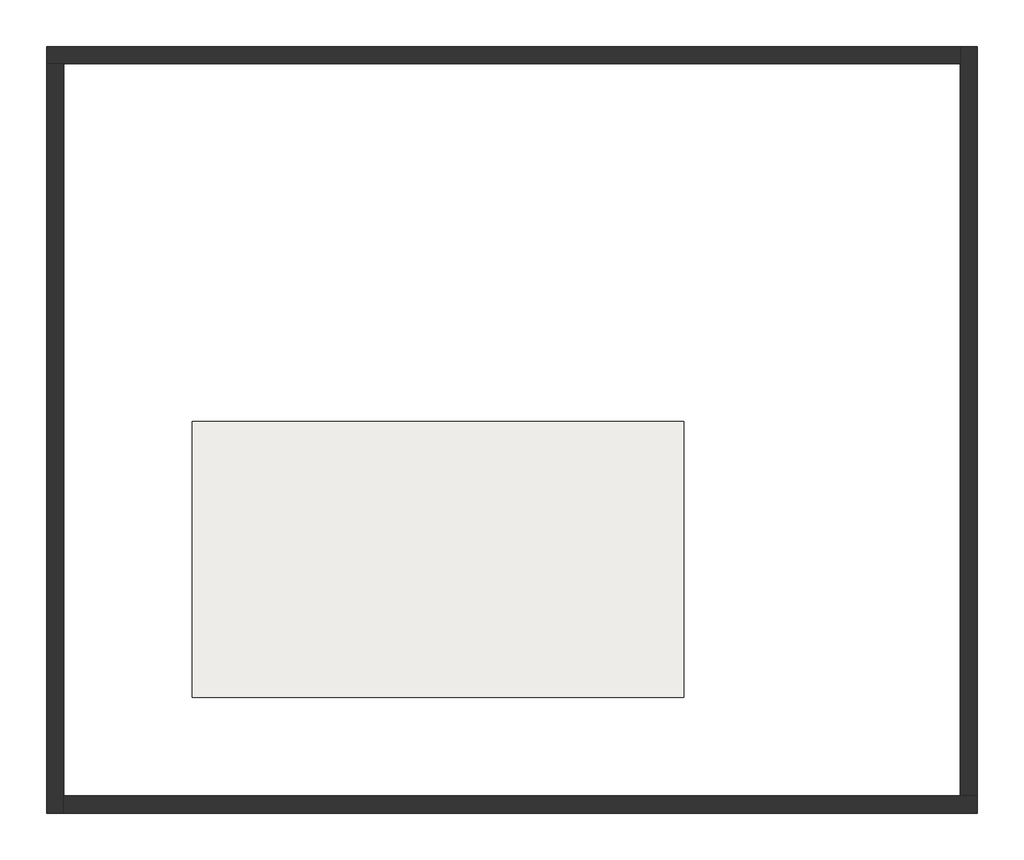
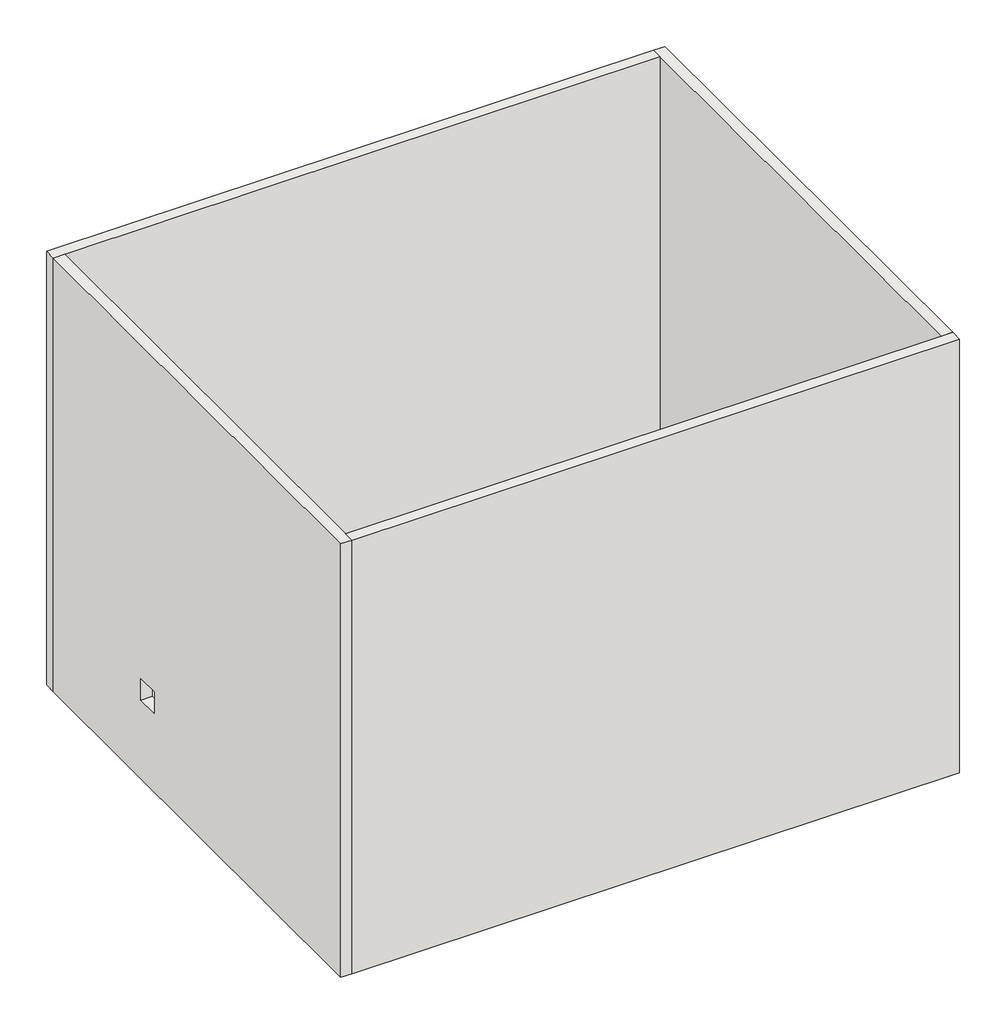
# One storey: 4 walls, 1 slab.
"""IFC4 building model written with IfcOpenShell, lengths in millimetres."""

import ifcopenshell
import ifcopenshell.guid

model = None  # the IFC model being written
_history = None  # IfcOwnerHistory: only IFC2X3 demands one
_inside = {}  # id of a spatial element -> (the spatial element, [elements in it])
_under = {}  # id of a project, library or spatial element -> (it, [spatial elements below it])
_declared = {}  # id of a project -> (the project, [libraries it declares])
_typed = {}  # id of a type object -> (the type object, [elements of that type])
_made_of = {}  # id of a material, layer set ... -> (it, [elements and type objects made of it])


def new_model(schema):
    """Start an empty IFC model of exactly this schema.

    Asked for "IFC4X3", IfcOpenShell would pick the latest addendum, in which some entities
    have other attributes; the version numbers below select the first issue.
    IFC2X3 requires an IfcOwnerHistory on every rooted entity: one is made here for all.
    """
    global model, _history
    if schema == "IFC4X3":
        model = ifcopenshell.file(schema_version=(4, 3, 0, 0))
    else:
        model = ifcopenshell.file(schema=schema)
    _inside.clear()
    _under.clear()
    _declared.clear()
    _typed.clear()
    _made_of.clear()
    _history = None
    if model.schema == "IFC2X3":
        org = make("IfcOrganization", Name="unknown")
        user = make(
            "IfcPersonAndOrganization",
            ThePerson=make("IfcPerson", FamilyName="unknown"),
            TheOrganization=org,
        )
        app = make(
            "IfcApplication",
            ApplicationDeveloper=org,
            Version="unknown",
            ApplicationFullName="unknown",
            ApplicationIdentifier="unknown",
        )
        _history = make(
            "IfcOwnerHistory",
            OwningUser=user,
            OwningApplication=app,
            ChangeAction="ADDED",
            CreationDate=0,
        )
    return model


def make(cls, **values):
    """One entity of the class cls with the attributes given. An attribute that is None is left unset."""
    return model.create_entity(
        cls, **{name: value for name, value in values.items() if value is not None}
    )


def rooted(cls, **values):
    """An entity with a GlobalId (a new one), such as an element, a storey or a relation."""
    return make(cls, GlobalId=ifcopenshell.guid.new(), OwnerHistory=_history, **values)


def si_unit(unit_type, name, prefix=None):
    """IfcSIUnit, for example si_unit("LENGTHUNIT", "METRE", prefix="MILLI")."""
    return make("IfcSIUnit", UnitType=unit_type, Prefix=prefix, Name=name)


def assignment(units):
    """IfcUnitAssignment: the units of a project."""
    return None if units is None else make("IfcUnitAssignment", Units=units)


def point(xyz):
    """IfcCartesianPoint."""
    return None if xyz is None else make("IfcCartesianPoint", Coordinates=xyz)


def direction(xyz):
    """IfcDirection."""
    return None if xyz is None else make("IfcDirection", DirectionRatios=xyz)


def frame(location, z_axis=None, x_axis=None):
    """IfcAxis2Placement3D, a coordinate frame: its origin and axes. An axis left out is left unset."""
    return make(
        "IfcAxis2Placement3D",
        Location=point(location),
        Axis=direction(z_axis),
        RefDirection=direction(x_axis),
    )


def origin():
    """The frame at (0, 0, 0) with its axes left unset."""
    return frame((0.0, 0.0, 0.0))


def place(relative_to, where):
    """IfcLocalPlacement: puts the frame where relative to a parent placement (None: the world)."""
    return make(
        "IfcLocalPlacement", PlacementRelTo=relative_to, RelativePlacement=where
    )


def context(
    kind, dimensions, precision=None, world=None, true_north=None, identifier=None
):
    """IfcGeometricRepresentationContext, for example the 3D "Model" context."""
    return make(
        "IfcGeometricRepresentationContext",
        ContextIdentifier=identifier,
        ContextType=kind,
        CoordinateSpaceDimension=dimensions,
        Precision=precision,
        WorldCoordinateSystem=world,
        TrueNorth=true_north,
    )


def project(units=None, contexts=None):
    """IfcProject with its units and contexts."""
    return rooted(
        "IfcProject",
        Name="project",
        RepresentationContexts=contexts,
        UnitsInContext=assignment(units),
    )


def spatial(cls, under=None, at=None, **own):
    """A site, building, storey or space (cls), placed at a placement, below another one or the project."""
    s = rooted(cls, ObjectPlacement=at, **own)
    if under is not None:
        _under.setdefault(under.id(), (under, []))[1].append(s)
    return s


def polyline(points):
    """IfcPolyline through the points."""
    return make("IfcPolyline", Points=[point(p) for p in points])


def outline(outer, holes=None, kind="AREA"):
    """IfcArbitraryClosedProfileDef: a profile drawn as a closed curve; with holes, ...WithVoids."""
    if holes is None:
        return make("IfcArbitraryClosedProfileDef", ProfileType=kind, OuterCurve=outer)
    return make(
        "IfcArbitraryProfileDefWithVoids",
        ProfileType=kind,
        OuterCurve=outer,
        InnerCurves=holes,
    )


def extrude(swept, where, along, depth):
    """IfcExtrudedAreaSolid: the profile swept, set in the frame where, extruded along a direction by depth."""
    return make(
        "IfcExtrudedAreaSolid",
        SweptArea=swept,
        Position=where,
        ExtrudedDirection=direction(along),
        Depth=depth,
    )


def faces_of(points, faces, orient=None, outer=None):
    """IfcFace entities. A face is a list of loops; a loop is a list of indices into points, from 0.

    orient and outer hold one flag for each loop. By default every Orientation is true, the
    first loop of a face is its IfcFaceOuterBound and the others are IfcFaceBound.
    """
    made = []
    for i, loops in enumerate(faces):
        bounds = []
        for j, loop in enumerate(loops):
            is_outer = j == 0 if outer is None else outer[i][j]
            bounds.append(
                make(
                    "IfcFaceOuterBound" if is_outer else "IfcFaceBound",
                    Bound=make("IfcPolyLoop", Polygon=[points[k] for k in loop]),
                    Orientation=True if orient is None else orient[i][j],
                )
            )
        made.append(make("IfcFace", Bounds=bounds))
    return made


def faceted_brep(points, faces, orient=None, outer=None, voids=None):
    """IfcFacetedBrep: a solid bounded by flat faces; with voids (closed shells), ...WithVoids."""
    shared = [point(p) for p in points]
    hull = make("IfcClosedShell", CfsFaces=faces_of(shared, faces, orient, outer))
    if voids is None:
        return make("IfcFacetedBrep", Outer=hull)
    return make(
        "IfcFacetedBrepWithVoids",
        Outer=hull,
        Voids=[
            make(cls, CfsFaces=faces_of(shared, fs, o, b)) for cls, fs, o, b in voids
        ],
    )


def shape(context_of_items, identifier, shape_type, items):
    """IfcShapeRepresentation: the items that make up one representation, for example the "Body"."""
    return make(
        "IfcShapeRepresentation",
        ContextOfItems=context_of_items,
        RepresentationIdentifier=identifier,
        RepresentationType=shape_type,
        Items=items,
    )


def made_of(thing, what):
    """Note that an element or type object is made of a material, layer set ...; save() writes the relation."""
    if what is not None:
        _made_of.setdefault(what.id(), (what, []))[1].append(thing)
    return thing


def element(
    cls,
    number,
    at=None,
    inside=None,
    cuts=None,
    type_object=None,
    material=None,
    context=None,
    identifier="Body",
    shape_type=None,
    held_by="IfcProductDefinitionShape",
    body=None,
    shapes=None,
    **own,
):
    """One element of the class cls, such as IfcWall. Its Tag is "e" and its number.

    at: its placement. inside: the storey or other place that contains it. cuts: it is an
    opening in that element (IfcRelVoidsElement). A single representation is given by context,
    identifier, shape_type and body (its items); several are given by shapes. held_by: the class
    of the entity that holds the representations. save() writes the other relations.
    """
    e = rooted(cls, Tag="e%d" % number, ObjectPlacement=at, **own)
    if body is not None:
        shapes = [shape(context, identifier, shape_type, body)]
    if shapes is not None:
        e.Representation = make(held_by, Representations=shapes)
    if inside is not None:
        _inside.setdefault(inside.id(), (inside, []))[1].append(e)
    if cuts is not None:
        rooted(
            "IfcRelVoidsElement", RelatingBuildingElement=cuts, RelatedOpeningElement=e
        )
    if type_object is not None:
        _typed.setdefault(type_object.id(), (type_object, []))[1].append(e)
    return made_of(e, material)


def aggregate(whole, parts):
    """IfcRelAggregates: a whole, such as a stair, and the parts it consists of."""
    return rooted("IfcRelAggregates", RelatingObject=whole, RelatedObjects=parts)


def save(model, path):
    """Write the relations noted so far, then the file.

    IfcRelAggregates (storeys below a building ...), IfcRelContainedInSpatialStructure (elements
    in a storey), IfcRelDefinesByType, IfcRelAssociatesMaterial and IfcRelDeclares: one each for
    every whole, place, type object, material and project.
    """
    for whole, parts in _under.values():
        aggregate(whole, parts)
    for where, things in _inside.values():
        rooted(
            "IfcRelContainedInSpatialStructure",
            RelatedElements=things,
            RelatingStructure=where,
        )
    for kind, things in _typed.values():
        rooted("IfcRelDefinesByType", RelatedObjects=things, RelatingType=kind)
    for what, things in _made_of.values():
        rooted("IfcRelAssociatesMaterial", RelatedObjects=things, RelatingMaterial=what)
    for by, libraries in _declared.values():
        rooted("IfcRelDeclares", RelatingContext=by, RelatedDefinitions=libraries)
    model.write(path)


model = new_model("IFC4")

# Units and contexts
model_context = context("Model", 3, world=origin())
ifc_project = project(units=[si_unit("LENGTHUNIT", "METRE", prefix="MILLI")], contexts=[model_context])

# Site, building, storey
site = spatial("IfcSite", under=ifc_project)
building = spatial("IfcBuilding", under=site)
storey = spatial("IfcBuildingStorey", under=building, Name="Уровень 1", Elevation=0.0)

# Slab
placement = place(None, origin())
element("IfcSlab", 1, ObjectType="Типовой 300мм", at=placement, inside=storey, context=model_context, shape_type="SweptSolid", body=[
    extrude(outline(polyline([(-708.4557777, 3404.1546212), (-708.4557777, 204.1546212), (-6408.4557777, 204.1546212), (-6408.4557777, 3404.1546212), (-708.4557777, 3404.1546212)])), frame((0.0, 0.0, -300.0), z_axis=(0.0, 0.0, 1.0), x_axis=(1.0, 0.0, 0.0)), (0.0, 0.0, 1.0), 300.0),
])

# Walls
element("IfcWall", 2, ObjectType="Типовой - 200мм", at=placement, inside=storey, context=model_context, shape_type="Brep", body=[
    faceted_brep([(-8101.7504428, 7556.494067, 0.0), (-7901.7504428, 7556.494067, 0.0), (2498.2495572, 7556.494067, 0.0), (2498.2495572, 7556.494067, 8000.0), (-7901.7504428, 7556.494067, 8000.0), (-8101.7504428, 7556.494067, 8000.0), (-8101.7504428, 7756.494067, 0.0), (-8101.7504428, 7756.494067, 8000.0), (2498.2495572, 7756.494067, 8000.0), (2498.2495572, 7756.494067, 0.0)], [[[0, 1, 2, 3, 4, 5]], [[6, 7, 8, 9]], [[2, 1, 0, 6, 9]], [[5, 4, 3, 8, 7]], [[0, 5, 7, 6]], [[3, 2, 9, 8]]]),
])
element("IfcWall", 3, ObjectType="Типовой - 200мм", at=placement, inside=storey, context=model_context, shape_type="Brep", body=[
    faceted_brep([(-7901.7504428, -1143.505933, 0.0), (-7901.7504428, -943.505933, 0.0), (-7901.7504428, 7556.494067, 0.0), (-7901.7504428, 7556.494067, 8000.0), (-7901.7504428, -943.505933, 8000.0), (-7901.7504428, -1143.505933, 8000.0), (-7901.7504428, 4501.8879995, 1850.0), (-7901.7504428, 4901.8879995, 1850.0), (-7901.7504428, 4901.8879995, 1450.0), (-7901.7504428, 4501.8879995, 1450.0), (-8101.7504428, 7556.494067, 0.0), (-8101.7504428, -1143.505933, 0.0), (-8101.7504428, -1143.505933, 8000.0), (-8101.7504428, 7556.494067, 8000.0), (-8101.7504428, 4901.8879995, 1850.0), (-8101.7504428, 4501.8879995, 1850.0), (-8101.7504428, 4501.8879995, 1450.0), (-8101.7504428, 4901.8879995, 1450.0)], [[[0, 1, 2, 3, 4, 5], [6, 7, 8, 9]], [[10, 11, 12, 13], [14, 15, 16, 17]], [[2, 1, 0, 11, 10]], [[5, 4, 3, 13, 12]], [[0, 5, 12, 11]], [[3, 2, 10, 13]], [[6, 15, 14, 7]], [[8, 17, 16, 9]], [[7, 14, 17, 8]], [[15, 6, 9, 16]]]),
])
element("IfcWall", 4, ObjectType="Типовой - 200мм", at=placement, inside=storey, context=model_context, shape_type="Brep", body=[
    faceted_brep([(2698.2495572, -943.505933, 0.0), (2498.2495572, -943.505933, 0.0), (-7901.7504428, -943.505933, 0.0), (-7901.7504428, -943.505933, 8000.0), (2498.2495572, -943.505933, 8000.0), (2698.2495572, -943.505933, 8000.0), (2698.2495572, -1143.505933, 0.0), (2698.2495572, -1143.505933, 8000.0), (-7901.7504428, -1143.505933, 8000.0), (-7901.7504428, -1143.505933, 0.0)], [[[0, 1, 2, 3, 4, 5]], [[6, 7, 8, 9]], [[2, 1, 0, 6, 9]], [[5, 4, 3, 8, 7]], [[0, 5, 7, 6]], [[3, 2, 9, 8]]]),
])
element("IfcWall", 5, ObjectType="Типовой - 200мм", at=placement, inside=storey, context=model_context, shape_type="Brep", body=[
    faceted_brep([(2498.2495572, 7756.494067, 0.0), (2498.2495572, 7556.494067, 0.0), (2498.2495572, -943.505933, 0.0), (2498.2495572, -943.505933, 8000.0), (2498.2495572, 7556.494067, 8000.0), (2498.2495572, 7756.494067, 8000.0), (2698.2495572, 7756.494067, 0.0), (2698.2495572, 7756.494067, 8000.0), (2698.2495572, -943.505933, 8000.0), (2698.2495572, -943.505933, 0.0)], [[[0, 1, 2, 3, 4, 5]], [[6, 7, 8, 9]], [[2, 1, 0, 6, 9]], [[5, 4, 3, 8, 7]], [[0, 5, 7, 6]], [[3, 2, 9, 8]]]),
])

save(model, "model.ifc")

# Revit data of these elements
# Project information
#   Дата утверждения проекта = "Дата выпуска"
#   Статус проекта = "Статус проекта"
#   Заказчик = "Владелец"
#   Адрес проекта = "Укажите адрес"
#   Наименование проекта = "Наименование проекта"
#   Номер проекта = "0001"
# Type "Типовой 300мм"
#   Function = 0
#   Layers, outside or top first: 300 mm no material (function 1)
# Type "Типовой - 200мм"
#   Layers, outside or top first: 200 mm no material (function 1)
# Element 1 (IfcSlab, "Типовой 300мм")
#   Height Offset From Level = 0 mm
#   Phase Created = Новая конструкция
#   Materials on its faces: "Этаж по умолчанию"
# Elements 2, 3, 4, 5 (IfcWall, "Типовой - 200мм")
#   Top Offset = 0 mm
#   Base Offset = 0 mm
#   Unconnected Height = 8000 mm
#   wall height = 8000 mm
#   Phase Created = Новая конструкция
#   Base Constraint = Уровень 1
#   Materials on its faces: "Стена по умолчанию"
# Materials
#   "Этаж по умолчанию": class "Разное", colour RGB 127 127 127, transparency 0, Cost = 0
#   "Стена по умолчанию": class "Разное", colour RGB 128 128 128, transparency 0, Cost = 0
